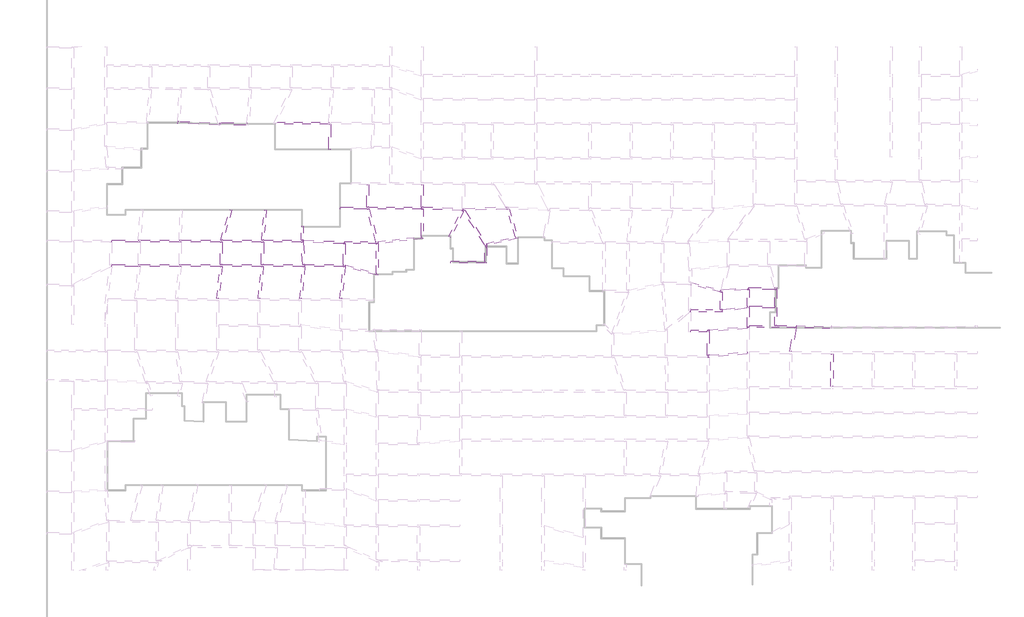
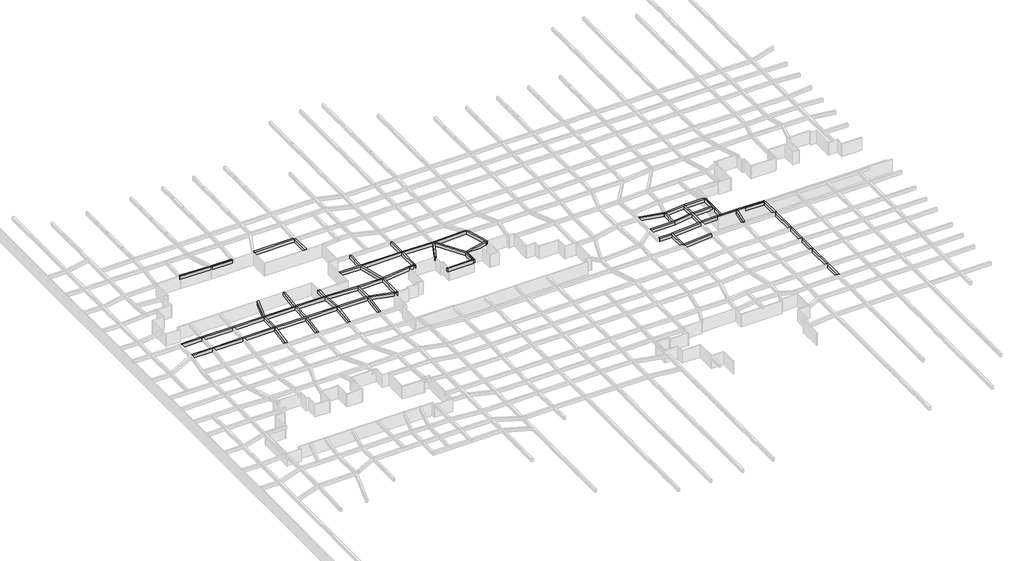
# One storey, part 30 of 45: 53 beams.
"""IFC4 building model written with IfcOpenShell, lengths in millimetres."""

import ifcopenshell
import ifcopenshell.guid

model = None  # the IFC model being written
_history = None  # IfcOwnerHistory: only IFC2X3 demands one
_inside = {}  # id of a spatial element -> (the spatial element, [elements in it])
_under = {}  # id of a project, library or spatial element -> (it, [spatial elements below it])
_declared = {}  # id of a project -> (the project, [libraries it declares])
_typed = {}  # id of a type object -> (the type object, [elements of that type])
_made_of = {}  # id of a material, layer set ... -> (it, [elements and type objects made of it])


def new_model(schema):
    """Start an empty IFC model of exactly this schema.

    Asked for "IFC4X3", IfcOpenShell would pick the latest addendum, in which some entities
    have other attributes; the version numbers below select the first issue.
    IFC2X3 requires an IfcOwnerHistory on every rooted entity: one is made here for all.
    """
    global model, _history
    if schema == "IFC4X3":
        model = ifcopenshell.file(schema_version=(4, 3, 0, 0))
    else:
        model = ifcopenshell.file(schema=schema)
    _inside.clear()
    _under.clear()
    _declared.clear()
    _typed.clear()
    _made_of.clear()
    _history = None
    if model.schema == "IFC2X3":
        org = make("IfcOrganization", Name="unknown")
        user = make(
            "IfcPersonAndOrganization",
            ThePerson=make("IfcPerson", FamilyName="unknown"),
            TheOrganization=org,
        )
        app = make(
            "IfcApplication",
            ApplicationDeveloper=org,
            Version="unknown",
            ApplicationFullName="unknown",
            ApplicationIdentifier="unknown",
        )
        _history = make(
            "IfcOwnerHistory",
            OwningUser=user,
            OwningApplication=app,
            ChangeAction="ADDED",
            CreationDate=0,
        )
    return model


def make(cls, **values):
    """One entity of the class cls with the attributes given. An attribute that is None is left unset."""
    return model.create_entity(
        cls, **{name: value for name, value in values.items() if value is not None}
    )


def rooted(cls, **values):
    """An entity with a GlobalId (a new one), such as an element, a storey or a relation."""
    return make(cls, GlobalId=ifcopenshell.guid.new(), OwnerHistory=_history, **values)


def si_unit(unit_type, name, prefix=None):
    """IfcSIUnit, for example si_unit("LENGTHUNIT", "METRE", prefix="MILLI")."""
    return make("IfcSIUnit", UnitType=unit_type, Prefix=prefix, Name=name)


def assignment(units):
    """IfcUnitAssignment: the units of a project."""
    return None if units is None else make("IfcUnitAssignment", Units=units)


def point(xyz):
    """IfcCartesianPoint."""
    return None if xyz is None else make("IfcCartesianPoint", Coordinates=xyz)


def direction(xyz):
    """IfcDirection."""
    return None if xyz is None else make("IfcDirection", DirectionRatios=xyz)


def frame(location, z_axis=None, x_axis=None):
    """IfcAxis2Placement3D, a coordinate frame: its origin and axes. An axis left out is left unset."""
    return make(
        "IfcAxis2Placement3D",
        Location=point(location),
        Axis=direction(z_axis),
        RefDirection=direction(x_axis),
    )


def origin():
    """The frame at (0, 0, 0) with its axes left unset."""
    return frame((0.0, 0.0, 0.0))


def place(relative_to, where):
    """IfcLocalPlacement: puts the frame where relative to a parent placement (None: the world)."""
    return make(
        "IfcLocalPlacement", PlacementRelTo=relative_to, RelativePlacement=where
    )


def context(
    kind, dimensions, precision=None, world=None, true_north=None, identifier=None
):
    """IfcGeometricRepresentationContext, for example the 3D "Model" context."""
    return make(
        "IfcGeometricRepresentationContext",
        ContextIdentifier=identifier,
        ContextType=kind,
        CoordinateSpaceDimension=dimensions,
        Precision=precision,
        WorldCoordinateSystem=world,
        TrueNorth=true_north,
    )


def project(units=None, contexts=None):
    """IfcProject with its units and contexts."""
    return rooted(
        "IfcProject",
        Name="project",
        RepresentationContexts=contexts,
        UnitsInContext=assignment(units),
    )


def spatial(cls, under=None, at=None, **own):
    """A site, building, storey or space (cls), placed at a placement, below another one or the project."""
    s = rooted(cls, ObjectPlacement=at, **own)
    if under is not None:
        _under.setdefault(under.id(), (under, []))[1].append(s)
    return s


def polyline(points):
    """IfcPolyline through the points."""
    return make("IfcPolyline", Points=[point(p) for p in points])


def outline(outer, holes=None, kind="AREA"):
    """IfcArbitraryClosedProfileDef: a profile drawn as a closed curve; with holes, ...WithVoids."""
    if holes is None:
        return make("IfcArbitraryClosedProfileDef", ProfileType=kind, OuterCurve=outer)
    return make(
        "IfcArbitraryProfileDefWithVoids",
        ProfileType=kind,
        OuterCurve=outer,
        InnerCurves=holes,
    )


def extrude(swept, where, along, depth):
    """IfcExtrudedAreaSolid: the profile swept, set in the frame where, extruded along a direction by depth."""
    return make(
        "IfcExtrudedAreaSolid",
        SweptArea=swept,
        Position=where,
        ExtrudedDirection=direction(along),
        Depth=depth,
    )


def faces_of(points, faces, orient=None, outer=None):
    """IfcFace entities. A face is a list of loops; a loop is a list of indices into points, from 0.

    orient and outer hold one flag for each loop. By default every Orientation is true, the
    first loop of a face is its IfcFaceOuterBound and the others are IfcFaceBound.
    """
    made = []
    for i, loops in enumerate(faces):
        bounds = []
        for j, loop in enumerate(loops):
            is_outer = j == 0 if outer is None else outer[i][j]
            bounds.append(
                make(
                    "IfcFaceOuterBound" if is_outer else "IfcFaceBound",
                    Bound=make("IfcPolyLoop", Polygon=[points[k] for k in loop]),
                    Orientation=True if orient is None else orient[i][j],
                )
            )
        made.append(make("IfcFace", Bounds=bounds))
    return made


def faceted_brep(points, faces, orient=None, outer=None, voids=None):
    """IfcFacetedBrep: a solid bounded by flat faces; with voids (closed shells), ...WithVoids."""
    shared = [point(p) for p in points]
    hull = make("IfcClosedShell", CfsFaces=faces_of(shared, faces, orient, outer))
    if voids is None:
        return make("IfcFacetedBrep", Outer=hull)
    return make(
        "IfcFacetedBrepWithVoids",
        Outer=hull,
        Voids=[
            make(cls, CfsFaces=faces_of(shared, fs, o, b)) for cls, fs, o, b in voids
        ],
    )


def shape(context_of_items, identifier, shape_type, items):
    """IfcShapeRepresentation: the items that make up one representation, for example the "Body"."""
    return make(
        "IfcShapeRepresentation",
        ContextOfItems=context_of_items,
        RepresentationIdentifier=identifier,
        RepresentationType=shape_type,
        Items=items,
    )


def made_of(thing, what):
    """Note that an element or type object is made of a material, layer set ...; save() writes the relation."""
    if what is not None:
        _made_of.setdefault(what.id(), (what, []))[1].append(thing)
    return thing


def element(
    cls,
    number,
    at=None,
    inside=None,
    cuts=None,
    type_object=None,
    material=None,
    context=None,
    identifier="Body",
    shape_type=None,
    held_by="IfcProductDefinitionShape",
    body=None,
    shapes=None,
    **own,
):
    """One element of the class cls, such as IfcWall. Its Tag is "e" and its number.

    at: its placement. inside: the storey or other place that contains it. cuts: it is an
    opening in that element (IfcRelVoidsElement). A single representation is given by context,
    identifier, shape_type and body (its items); several are given by shapes. held_by: the class
    of the entity that holds the representations. save() writes the other relations.
    """
    e = rooted(cls, Tag="e%d" % number, ObjectPlacement=at, **own)
    if body is not None:
        shapes = [shape(context, identifier, shape_type, body)]
    if shapes is not None:
        e.Representation = make(held_by, Representations=shapes)
    if inside is not None:
        _inside.setdefault(inside.id(), (inside, []))[1].append(e)
    if cuts is not None:
        rooted(
            "IfcRelVoidsElement", RelatingBuildingElement=cuts, RelatedOpeningElement=e
        )
    if type_object is not None:
        _typed.setdefault(type_object.id(), (type_object, []))[1].append(e)
    return made_of(e, material)


def aggregate(whole, parts):
    """IfcRelAggregates: a whole, such as a stair, and the parts it consists of."""
    return rooted("IfcRelAggregates", RelatingObject=whole, RelatedObjects=parts)


def save(model, path):
    """Write the relations noted so far, then the file.

    IfcRelAggregates (storeys below a building ...), IfcRelContainedInSpatialStructure (elements
    in a storey), IfcRelDefinesByType, IfcRelAssociatesMaterial and IfcRelDeclares: one each for
    every whole, place, type object, material and project.
    """
    for whole, parts in _under.values():
        aggregate(whole, parts)
    for where, things in _inside.values():
        rooted(
            "IfcRelContainedInSpatialStructure",
            RelatedElements=things,
            RelatingStructure=where,
        )
    for kind, things in _typed.values():
        rooted("IfcRelDefinesByType", RelatedObjects=things, RelatingType=kind)
    for what, things in _made_of.values():
        rooted("IfcRelAssociatesMaterial", RelatedObjects=things, RelatingMaterial=what)
    for by, libraries in _declared.values():
        rooted("IfcRelDeclares", RelatingContext=by, RelatedDefinitions=libraries)
    model.write(path)


model = new_model("IFC4")

# Units and contexts
model_context = context("Model", 3, world=origin())
ifc_project = project(units=[si_unit("LENGTHUNIT", "METRE", prefix="MILLI")], contexts=[model_context])

# Site, building, storey
site = spatial("IfcSite", under=ifc_project)
building = spatial("IfcBuilding", under=site)
storey = spatial("IfcBuildingStorey", under=building, Name="户型图", Elevation=0.0)

# Beams
placement = place(None, origin())
element("IfcBeam", 1, ObjectType="混凝土 - 矩形梁 : KL_beam", at=placement, inside=storey, context=model_context, shape_type="Brep", body=[
    faceted_brep([(-106255.594098, 67607.285668, 3300.0), (-106259.7681682, 67607.285668, 3300.0), (-106661.2961032, 67607.285668, 3300.0), (-114062.8131158, 67607.285668, 3300.0), (-114464.9837666, 67607.285668, 3300.0), (-121862.8299892, 67607.285668, 3300.0), (-122265.00064, 67607.285668, 3300.0), (-129662.8131158, 67607.285668, 3300.0), (-130064.9837666, 67607.285668, 3300.0), (-137362.8299892, 67607.285668, 3300.0), (-137765.00064, 67607.285668, 3300.0), (-142766.12907, 67607.285668, 3300.0), (-142895.0186512, 67607.285668, 3300.0), (-142895.0186512, 67607.285668, 2500.0), (-142766.12907, 67607.285668, 2500.0), (-137765.00064, 67607.285668, 2500.0), (-137362.8299892, 67607.285668, 2500.0), (-130064.9837666, 67607.285668, 2500.0), (-129662.8131158, 67607.285668, 2500.0), (-122265.00064, 67607.285668, 2500.0), (-121862.8299892, 67607.285668, 2500.0), (-114464.9837666, 67607.285668, 2500.0), (-114062.8131158, 67607.285668, 2500.0), (-106661.2961032, 67607.285668, 2500.0), (-106259.7681682, 67607.285668, 2500.0), (-106255.594098, 67607.285668, 2500.0), (-142743.034403, 67684.7255104, 3300.0), (-142743.034403, 67684.7255104, 2500.0), (-142743.034403, 68007.285668, 3300.0), (-142743.034403, 68007.285668, 2500.0), (-106255.594098, 68007.285668, 3300.0), (-106656.4356776, 68007.285668, 3300.0), (-114043.034403, 68007.285668, 3300.0), (-114443.034403, 68007.285668, 3300.0), (-121843.034403, 68007.285668, 3300.0), (-122243.034403, 68007.285668, 3300.0), (-129643.034403, 68007.285668, 3300.0), (-130043.034403, 68007.285668, 3300.0), (-137343.034403, 68007.285668, 3300.0), (-137743.034403, 68007.285668, 3300.0), (-137743.034403, 68007.285668, 2500.0), (-137343.034403, 68007.285668, 2500.0), (-130043.034403, 68007.285668, 2500.0), (-129643.034403, 68007.285668, 2500.0), (-122243.034403, 68007.285668, 2500.0), (-121843.034403, 68007.285668, 2500.0), (-114443.034403, 68007.285668, 2500.0), (-114043.034403, 68007.285668, 2500.0), (-106656.4356776, 68007.285668, 2500.0), (-106255.594098, 68007.285668, 2500.0)], [[[0, 1, 2, 3, 4, 5, 6, 7, 8, 9, 10, 11, 12, 13, 14, 15, 16, 17, 18, 19, 20, 21, 22, 23, 24, 25]], [[26, 27, 13, 12]], [[27, 26, 28, 29]], [[30, 31, 32, 33, 34, 35, 36, 37, 38, 39, 28, 26, 12, 11, 10, 9, 8, 7, 6, 5, 4, 3, 2, 1, 0]], [[25, 24, 23, 22, 21, 20, 19, 18, 17, 16, 15, 14, 13, 27, 29, 40, 41, 42, 43, 44, 45, 46, 47, 48, 49]], [[28, 39, 38, 37, 36, 35, 34, 33, 32, 31, 30, 49, 48, 47, 46, 45, 44, 43, 42, 41, 40, 29]], [[30, 0, 25, 49]]]),
])
element("IfcBeam", 2, ObjectType="混凝土 - 矩形梁 : KL_beam", at=placement, inside=storey, context=model_context, shape_type="Brep", body=[
    faceted_brep([(-142743.034403, 72629.6091605, 3300.0), (-142743.034403, 72229.932653, 3300.0), (-142743.034403, 72229.6091605, 3300.0), (-137743.034403, 72229.6091605, 3300.0), (-137343.034403, 72229.6091605, 3300.0), (-130043.034403, 72229.6091605, 3300.0), (-129643.034403, 72229.6091605, 3300.0), (-122243.034403, 72229.6091605, 3300.0), (-121843.034403, 72229.6091605, 3300.0), (-114443.034403, 72229.6091605, 3300.0), (-114043.034403, 72229.6091605, 3300.0), (-106930.474708, 72229.6091605, 3300.0), (-106529.6331284, 72229.6091605, 3300.0), (-106543.0328284, 72436.0683208, 3300.0), (-106555.594098, 72629.6091605, 3300.0), (-106943.0328284, 72629.6091605, 3300.0), (-114024.7727028, 72629.6091605, 3300.0), (-114426.3006378, 72629.6091605, 3300.0), (-121772.7499154, 72629.6091605, 3300.0), (-122191.026618, 72629.6091605, 3300.0), (-129635.9283402, 72629.6091605, 3300.0), (-130036.172158, 72629.6091605, 3300.0), (-137328.560661, 72629.6091605, 3300.0), (-137729.5374202, 72629.6091605, 3300.0), (-106529.6331284, 72229.6091605, 2500.0), (-142743.034403, 72229.6091605, 2500.0), (-137743.034403, 72229.6091605, 2500.0), (-137343.034403, 72229.6091605, 2500.0), (-130043.034403, 72229.6091605, 2500.0), (-129643.034403, 72229.6091605, 2500.0), (-122243.034403, 72229.6091605, 2500.0), (-121843.034403, 72229.6091605, 2500.0), (-114443.034403, 72229.6091605, 2500.0), (-114043.034403, 72229.6091605, 2500.0), (-106930.474708, 72229.6091605, 2500.0), (-142743.034403, 72229.932653, 2500.0), (-142743.034403, 72629.6091605, 2500.0), (-137729.5374202, 72629.6091605, 2500.0), (-137328.560661, 72629.6091605, 2500.0), (-130036.172158, 72629.6091605, 2500.0), (-129635.9283402, 72629.6091605, 2500.0), (-122191.026618, 72629.6091605, 2500.0), (-121772.7499154, 72629.6091605, 2500.0), (-114426.3006378, 72629.6091605, 2500.0), (-114024.7727028, 72629.6091605, 2500.0), (-106943.0328284, 72629.6091605, 2500.0), (-106555.594098, 72629.6091605, 2500.0), (-106543.0328284, 72436.0683208, 2500.0)], [[[0, 1, 2, 3, 4, 5, 6, 7, 8, 9, 10, 11, 12, 13, 14, 15, 16, 17, 18, 19, 20, 21, 22, 23]], [[24, 12, 11, 10, 9, 8, 7, 6, 5, 4, 3, 2, 25, 26, 27, 28, 29, 30, 31, 32, 33, 34]], [[25, 35, 36, 37, 38, 39, 40, 41, 42, 43, 44, 45, 46, 47, 24, 34, 33, 32, 31, 30, 29, 28, 27, 26]], [[36, 0, 23, 22, 21, 20, 19, 18, 17, 16, 15, 14, 46, 45, 44, 43, 42, 41, 40, 39, 38, 37]], [[0, 36, 35, 25, 2, 1]], [[14, 13, 12, 24, 47, 46]]]),
])
element("IfcBeam", 3, ObjectType="混凝土 - 矩形梁 : KL_beam", at=placement, inside=storey, context=model_context, shape_type="SweptSolid", body=[
    extrude(outline(polyline([(-121843.034403, 68007.285668), (-122243.034403, 68007.285668), (-122243.034403, 72229.6091605), (-121843.034403, 72229.6091605), (-121843.034403, 68007.285668)])), frame((0.0, 0.0, 2500.0), z_axis=(0.0, 0.0, 1.0), x_axis=(1.0, 0.0, 0.0)), (0.0, 0.0, 1.0), 800.0),
])
element("IfcBeam", 4, ObjectType="混凝土 - 矩形梁 : KL_beam", at=placement, inside=storey, context=model_context, shape_type="SweptSolid", body=[
    extrude(outline(polyline([(-114043.034403, 68007.285668), (-114443.034403, 68007.285668), (-114443.034403, 72229.6091605), (-114043.034403, 72229.6091605), (-114043.034403, 68007.285668)])), frame((0.0, 0.0, 2500.0), z_axis=(0.0, 0.0, 1.0), x_axis=(1.0, 0.0, 0.0)), (0.0, 0.0, 1.0), 800.0),
])
element("IfcBeam", 5, ObjectType="混凝土 - 矩形梁 : KL_beam", at=placement, inside=storey, context=model_context, shape_type="Brep", body=[
    faceted_brep([(-106656.4356776, 68007.285668, 3300.0), (-106255.594098, 68007.285668, 3300.0), (-106529.1388631, 72221.9936481, 3300.0), (-106529.6331284, 72229.6091605, 3300.0), (-106930.474708, 72229.6091605, 3300.0), (-106229.6331284, 67607.285668, 3300.0), (-106229.6331284, 67607.285668, 2500.0), (-106255.594098, 68007.285668, 2500.0), (-106529.1388631, 72221.9936481, 2500.0), (-106529.6331284, 72229.6091605, 2500.0), (-106656.4356776, 68007.285668, 2500.0), (-106930.474708, 72229.6091605, 2500.0), (-106255.594098, 67607.285668, 3300.0), (-106255.594098, 67607.285668, 2500.0)], [[[0, 1, 2, 3, 4]], [[5, 6, 7, 8, 9, 3, 2, 1]], [[7, 10, 11, 9, 8]], [[10, 0, 4, 11]], [[6, 5, 12, 13]], [[7, 1, 0, 10]], [[1, 7, 13, 12]], [[12, 5, 1]], [[6, 13, 7]], [[4, 3, 9, 11]]]),
])
element("IfcBeam", 6, ObjectType="混凝土 - 矩形梁 : KL_beam", at=placement, inside=storey, context=model_context, shape_type="SweptSolid", body=[
    extrude(outline(polyline([(-120421.5907849, 78417.1729884), (-120039.0688825, 78300.2243065), (-121772.7499154, 72629.6091605), (-122191.026618, 72629.6091605), (-120421.5907849, 78417.1729884)])), frame((0.0, 0.0, 2500.0), z_axis=(0.0, 0.0, 1.0), x_axis=(1.0, 0.0, 0.0)), (0.0, 0.0, 1.0), 800.0),
])
element("IfcBeam", 7, ObjectType="混凝土 - 矩形梁 : KL_beam", at=placement, inside=storey, context=model_context, shape_type="SweptSolid", body=[
    extrude(outline(polyline([(-113928.0544604, 78324.5890278), (-113529.5765812, 78289.7267307), (-114024.7727028, 72629.6091605), (-114426.3006378, 72629.6091605), (-113928.0544604, 78324.5890278)])), frame((0.0, 0.0, 2500.0), z_axis=(0.0, 0.0, 1.0), x_axis=(1.0, 0.0, 0.0)), (0.0, 0.0, 1.0), 800.0),
])
element("IfcBeam", 8, ObjectType="混凝土 - 矩形梁 : KL_beam", at=placement, inside=storey, context=model_context, shape_type="Brep", body=[
    faceted_brep([(-106943.0328284, 75329.5848988, 3300.0), (-106543.0328284, 75329.5848988, 3300.0), (-106543.0328284, 75329.5848988, 2500.0), (-106943.0328284, 75329.5848988, 2500.0), (-106943.0328284, 72629.6091605, 3300.0), (-106555.594098, 72629.6091605, 3300.0), (-106543.0328284, 72436.0683208, 3300.0), (-106543.0328284, 72622.7226537, 3300.0), (-106543.0328284, 72436.0683208, 2500.0), (-106543.0328284, 72622.7226537, 2500.0), (-106555.594098, 72629.6091605, 2500.0), (-106943.0328284, 72629.6091605, 2500.0)], [[[0, 1, 2, 3]], [[1, 0, 4, 5, 6, 7]], [[2, 1, 7, 6, 8, 9]], [[3, 2, 9, 8, 10, 11]], [[0, 3, 11, 4]], [[5, 10, 8, 6]], [[10, 5, 4, 11]]]),
])
element("IfcBeam", 9, ObjectType="混凝土 - 矩形梁 : KL_beam", at=placement, inside=storey, context=model_context, shape_type="SweptSolid", body=[
    extrude(outline(polyline([(-111770.1722019, 94559.1732079), (-111583.6491387, 94959.1732079), (-101725.1277611, 94959.1732079), (-101753.0984859, 94559.1732079), (-111770.1722019, 94559.1732079)])), frame((0.0, 0.0, 2500.0), z_axis=(0.0, 0.0, 1.0), x_axis=(1.0, 0.0, 0.0)), (0.0, 0.0, 1.0), 800.0),
])
element("IfcBeam", 10, ObjectType="混凝土 - 矩形梁 : KL_beam", at=placement, inside=storey, context=model_context, shape_type="Brep", body=[
    faceted_brep([(-101338.6349683, 89759.1001002, 3300.0), (-101738.6349683, 89759.1001002, 3300.0), (-101738.6349683, 89759.1001002, 2500.0), (-101338.6349683, 89759.1001002, 2500.0), (-101338.6349683, 94559.0757309, 3300.0), (-101352.1285421, 94559.0790192, 3300.0), (-101738.6349683, 94559.1732079, 3300.0), (-101738.6349683, 94559.1732079, 2500.0), (-101352.1285421, 94559.0790192, 2500.0), (-101338.6349683, 94559.0757309, 2500.0)], [[[0, 1, 2, 3]], [[1, 0, 4, 5, 6]], [[2, 1, 6, 7]], [[3, 2, 7, 8, 9]], [[0, 3, 9, 4]], [[4, 9, 8, 7, 6, 5]]]),
])
element("IfcBeam", 11, ObjectType="混凝土 - 矩形梁 : KL_beam", at=placement, inside=storey, context=model_context, shape_type="SweptSolid", body=[
    extrude(outline(polyline([(-122119.8995169, 94446.2535162), (-122242.1917895, 94846.2535162), (-117187.4621963, 94846.2535162), (-117215.4329211, 94446.2535162), (-122119.8995169, 94446.2535162)])), frame((0.0, 0.0, 2500.0), z_axis=(0.0, 0.0, 1.0), x_axis=(1.0, 0.0, 0.0)), (0.0, 0.0, 1.0), 800.0),
])
element("IfcBeam", 12, ObjectType="混凝土 - 矩形梁 : KL_beam", at=placement, inside=storey, context=model_context, shape_type="Brep", body=[
    faceted_brep([(-122397.9223476, 94446.3883014, 3300.0), (-122397.9223476, 94446.3883014, 2500.0), (-122383.9625489, 94846.1446322, 2500.0), (-122383.9625489, 94846.1446322, 3300.0), (-129850.782274, 95106.8917227, 3300.0), (-130250.5386048, 95120.8515214, 3300.0), (-130264.4984035, 94721.0951906, 3300.0), (-129850.782274, 95106.8917227, 2500.0), (-130250.5386048, 95120.8515214, 2500.0), (-130264.4984035, 94721.0951906, 2500.0)], [[[0, 1, 2, 3]], [[0, 3, 4, 5, 6]], [[3, 2, 7, 8, 5, 4]], [[2, 1, 9, 8, 7]], [[1, 0, 6, 9]], [[6, 5, 8, 9]]]),
])
element("IfcBeam", 13, ObjectType="混凝土 - 矩形梁 : KL_beam", at=placement, inside=storey, context=model_context, shape_type="Brep", body=[
    faceted_brep([(-76269.0646381, 78646.8472266, 3300.0), (-76269.0646381, 78246.6034089, 3300.0), (-75912.1939504, 78259.0656079, 3300.0), (-68020.5737025, 78534.6470595, 3300.0), (-67874.1816912, 78539.7591812, 3300.0), (-67874.1816912, 78940.0029989, 3300.0), (-68231.227169, 78927.5346961, 3300.0), (-76029.0040152, 78655.2303283, 3300.0), (-76269.0646381, 78646.8472266, 2500.0), (-67874.1816912, 78940.0029989, 2500.0), (-68231.227169, 78927.5346961, 2500.0), (-76029.0040152, 78655.2303283, 2500.0), (-76269.0646381, 78246.6034089, 2500.0), (-67874.1816912, 78539.7591812, 2500.0), (-68020.5737025, 78534.6470595, 2500.0), (-75912.1939504, 78259.0656079, 2500.0)], [[[0, 1, 2, 3, 4, 5, 6, 7]], [[8, 0, 7, 6, 5, 9, 10, 11]], [[12, 8, 11, 10, 9, 13, 14, 15]], [[1, 12, 15, 14, 13, 4, 3, 2]], [[4, 13, 9, 5]], [[1, 0, 8, 12]]]),
])
element("IfcBeam", 14, ObjectType="混凝土 - 矩形梁 : KL_beam", at=placement, inside=storey, context=model_context, shape_type="Brep", body=[
    faceted_brep([(-76269.0646381, 78246.6034089, 3300.0), (-76269.0646381, 78646.8472266, 3300.0), (-76429.0040152, 78652.4324327, 3300.0), (-83861.6804358, 78911.9872127, 3300.0), (-84261.6804358, 78925.9555205, 3300.0), (-84261.6804358, 78918.8494577, 3300.0), (-84261.6804358, 78525.7117028, 3300.0), (-84065.1714488, 78518.8494577, 3300.0), (-83862.0339972, 78511.7557416, 3300.0), (-76584.1894618, 78257.6078102, 3300.0), (-76381.2779443, 78250.5219839, 3300.0), (-76269.0646381, 78646.8472266, 2500.0), (-76429.0040152, 78652.4324327, 2500.0), (-83861.6804358, 78911.9872127, 2500.0), (-84261.6804358, 78925.9555205, 2500.0), (-76269.0646381, 78246.6034089, 2500.0), (-76381.2779443, 78250.5219839, 2500.0), (-76584.1894618, 78257.6078102, 2500.0), (-83862.0339972, 78511.7557416, 2500.0), (-84065.1714488, 78518.8494577, 2500.0), (-84261.6804358, 78525.7117028, 2500.0), (-84261.6804358, 78918.8494577, 2500.0)], [[[0, 1, 2, 3, 4, 5, 6, 7, 8, 9, 10]], [[1, 11, 12, 13, 14, 4, 3, 2]], [[11, 15, 16, 17, 18, 19, 20, 21, 14, 13, 12]], [[15, 0, 10, 9, 8, 7, 6, 20, 19, 18, 17, 16]], [[0, 15, 11, 1]], [[6, 5, 4, 14, 21, 20]]]),
])
element("IfcBeam", 15, ObjectType="混凝土 - 矩形梁 : KL_beam", at=placement, inside=storey, context=model_context, shape_type="SweptSolid", body=[
    extrude(outline(polyline([(-83861.6804358, 78911.9872127), (-84261.6804358, 78925.9555205), (-84261.6804358, 83154.2865852), (-83861.6804358, 83154.2865852), (-83861.6804358, 78911.9872127)])), frame((0.0, 0.0, 2500.0), z_axis=(0.0, 0.0, 1.0), x_axis=(1.0, 0.0, 0.0)), (0.0, 0.0, 1.0), 800.0),
])
element("IfcBeam", 16, ObjectType="混凝土 - 矩形梁 : KL_beam", at=placement, inside=storey, context=model_context, shape_type="Brep", body=[
    faceted_brep([(-99591.0339972, 78518.8494577, 3300.0), (-99591.0339972, 78918.8494577, 3300.0), (-99591.0339972, 78918.8494577, 2500.0), (-99591.0339972, 78518.8494577, 2500.0), (-94484.7943922, 78518.8494577, 3300.0), (-94070.68392, 78518.8494577, 3300.0), (-84262.0339972, 78518.8494577, 3300.0), (-84065.1714488, 78518.8494577, 3300.0), (-84261.6804358, 78525.7117028, 3300.0), (-84261.6804358, 78918.8494577, 3300.0), (-94131.3875586, 78918.8494577, 3300.0), (-94531.3875586, 78918.8494577, 3300.0), (-84261.6804358, 78918.8494577, 2500.0), (-94131.3875586, 78918.8494577, 2500.0), (-94531.3875586, 78918.8494577, 2500.0), (-84261.6804358, 78525.7117028, 2500.0), (-84065.1714488, 78518.8494577, 2500.0), (-84262.0339972, 78518.8494577, 2500.0), (-94070.68392, 78518.8494577, 2500.0), (-94484.7943922, 78518.8494577, 2500.0)], [[[0, 1, 2, 3]], [[1, 0, 4, 5, 6, 7, 8, 9, 10, 11]], [[2, 1, 11, 10, 9, 12, 13, 14]], [[3, 2, 14, 13, 12, 15, 16, 17, 18, 19]], [[0, 3, 19, 18, 17, 16, 7, 6, 5, 4]], [[15, 8, 7, 16]], [[8, 15, 12, 9]]]),
])
element("IfcBeam", 17, ObjectType="混凝土 - 矩形梁 : KL_beam", at=placement, inside=storey, context=model_context, shape_type="SweptSolid", body=[
    extrude(outline(polyline([(-94531.3875586, 83154.2865852), (-94131.3875586, 83154.2865852), (-94131.3875586, 78918.8494577), (-94531.3875586, 78918.8494577), (-94531.3875586, 83154.2865852)])), frame((0.0, 0.0, 2500.0), z_axis=(0.0, 0.0, 1.0), x_axis=(1.0, 0.0, 0.0)), (0.0, 0.0, 1.0), 800.0),
])
element("IfcBeam", 18, ObjectType="混凝土 - 矩形梁 : KL_beam", at=placement, inside=storey, context=model_context, shape_type="Brep", body=[
    faceted_brep([(-29976.7146993, 50850.070339, 3300.0), (-29959.2503222, 50450.070339, 3300.0), (-29767.9825107, 50466.8041042, 3300.0), (-22564.0859234, 51097.0633889, 3300.0), (-22564.0859234, 51498.5913239, 3300.0), (-29767.9825107, 50868.3320393, 3300.0), (-29959.2503222, 50450.070339, 2500.0), (-29767.9825107, 50466.8041042, 2500.0), (-22564.0859234, 51097.0633889, 2500.0), (-29976.7146993, 50850.070339, 2500.0), (-29767.9825107, 50868.3320393, 2500.0), (-22564.0859234, 51498.5913239, 2500.0)], [[[0, 1, 2, 3, 4, 5]], [[1, 6, 7, 8, 3, 2]], [[6, 9, 10, 11, 8, 7]], [[9, 0, 5, 4, 11, 10]], [[0, 9, 6, 1]], [[4, 3, 8, 11]]]),
])
element("IfcBeam", 19, ObjectType="混凝土 - 矩形梁 : KL_beam", at=placement, inside=storey, context=model_context, shape_type="Brep", body=[
    faceted_brep([(-30167.9825107, 50850.070339, 3300.0), (-29976.7146993, 50850.070339, 3300.0), (-29767.9825107, 50868.3320393, 3300.0), (-29767.9825107, 55266.8041042, 3300.0), (-29767.9825107, 55650.070339, 3300.0), (-29976.7146993, 55650.070339, 3300.0), (-30167.9825107, 55650.070339, 3300.0), (-30167.9825107, 55250.070339, 3300.0), (-29767.9825107, 55650.070339, 2500.0), (-29767.9825107, 50868.3320393, 2500.0), (-29767.9825107, 55266.8041042, 2500.0), (-29976.7146993, 50850.070339, 2500.0), (-30167.9825107, 50850.070339, 2500.0), (-30167.9825107, 55250.070339, 2500.0), (-30167.9825107, 55650.070339, 2500.0), (-29976.7146993, 55650.070339, 2500.0)], [[[0, 1, 2, 3, 4, 5, 6, 7]], [[8, 4, 3, 2, 9, 10]], [[11, 12, 13, 14, 15, 8, 10, 9]], [[12, 0, 7, 6, 14, 13]], [[1, 0, 12, 11]], [[2, 1, 11, 9]], [[6, 5, 4, 8, 15, 14]]]),
])
element("IfcBeam", 20, ObjectType="混凝土 - 矩形梁 : KL_beam", at=placement, inside=storey, context=model_context, shape_type="Brep", body=[
    faceted_brep([(-65916.2620344, 73019.8751777, 3300.0), (-67600.9427374, 78530.2174666, 3300.0), (-67874.1816912, 78539.7591812, 3300.0), (-67981.3269257, 78536.0175871, 3300.0), (-68020.5737025, 78534.6470595, 3300.0), (-66416.0181954, 73286.3824777, 3300.0), (-66298.7839367, 72902.9264958, 3300.0), (-68020.5737025, 78534.6470595, 2500.0), (-66416.0181954, 73286.3824777, 2500.0), (-66298.7839367, 72902.9264958, 2500.0), (-67600.9427374, 78530.2174666, 2500.0), (-65916.2620344, 73019.8751777, 2500.0), (-67981.3269257, 78536.0175871, 2500.0), (-67874.1816912, 78539.7591812, 2500.0)], [[[0, 1, 2, 3, 4, 5, 6]], [[6, 5, 4, 7, 8, 9]], [[10, 11, 9, 8, 7, 12, 13]], [[1, 0, 11, 10]], [[2, 1, 10, 13]], [[7, 4, 3, 2, 13, 12]], [[0, 6, 9, 11]]]),
])
element("IfcBeam", 21, ObjectType="混凝土 - 矩形梁 : KL_beam", at=placement, inside=storey, context=model_context, shape_type="Brep", body=[
    faceted_brep([(-76269.0646381, 78246.6034089, 3300.0), (-76381.2779443, 78250.5219839, 3300.0), (-76245.9854172, 78038.560049, 3300.0), (-72218.8192159, 71729.2245821, 3300.0), (-71818.8192159, 71102.5471468, 3300.0), (-71818.8192159, 71628.5259359, 3300.0), (-71818.8192159, 71846.0016564, 3300.0), (-71926.2124219, 72014.2539038, 3300.0), (-75912.1939504, 78259.0656079, 3300.0), (-76029.0040152, 78254.9865105, 3300.0), (-76381.2779443, 78250.5219839, 2500.0), (-76245.9854172, 78038.560049, 2500.0), (-72218.8192159, 71729.2245821, 2500.0), (-71818.8192159, 71102.5471468, 2500.0), (-76269.0646381, 78246.6034089, 2500.0), (-76029.0040152, 78254.9865105, 2500.0), (-75912.1939504, 78259.0656079, 2500.0), (-71926.2124219, 72014.2539038, 2500.0), (-71818.8192159, 71846.0016564, 2500.0), (-71818.8192159, 71628.5259359, 2500.0)], [[[0, 1, 2, 3, 4, 5, 6, 7, 8, 9]], [[1, 10, 11, 12, 13, 4, 3, 2]], [[10, 14, 15, 16, 17, 18, 19, 13, 12, 11]], [[16, 8, 7, 6, 18, 17]], [[1, 0, 14, 10]], [[8, 16, 15, 14, 0, 9]], [[6, 5, 4, 13, 19, 18]]]),
])
element("IfcBeam", 22, ObjectType="混凝土 - 矩形梁 : KL_beam", at=placement, inside=storey, context=model_context, shape_type="Brep", body=[
    faceted_brep([(-72218.8192159, 68287.6131193, 3300.0), (-71818.8192159, 68287.6131193, 3300.0), (-71818.8192159, 71102.5471468, 3300.0), (-72218.8192159, 71729.2245821, 3300.0), (-72218.8192159, 68687.6131193, 3300.0), (-72218.8192159, 68287.6131193, 2500.0), (-72218.8192159, 71729.2245821, 2500.0), (-72218.8192159, 68687.6131193, 2500.0), (-71818.8192159, 68287.6131193, 2500.0), (-71818.8192159, 71102.5471468, 2500.0)], [[[0, 1, 2, 3, 4]], [[5, 0, 4, 3, 6, 7]], [[8, 5, 7, 6, 9]], [[1, 8, 9, 2]], [[3, 2, 9, 6]], [[1, 0, 5, 8]]]),
])
element("IfcBeam", 23, ObjectType="混凝土 - 矩形梁 : KL_beam", at=placement, inside=storey, context=model_context, shape_type="SweptSolid", body=[
    extrude(outline(polyline([(-78618.8192159, 68287.6131193), (-78618.8192159, 68687.6131193), (-72218.8192159, 68687.6131193), (-72218.8192159, 68287.6131193), (-78618.8192159, 68287.6131193)])), frame((0.0, 0.0, 2500.0), z_axis=(0.0, 0.0, 1.0), x_axis=(1.0, 0.0, 0.0)), (0.0, 0.0, 1.0), 800.0),
])
element("IfcBeam", 24, ObjectType="混凝土 - 矩形梁 : KL_beam", at=placement, inside=storey, context=model_context, shape_type="Brep", body=[
    faceted_brep([(-84262.0339972, 72894.8122003, 3300.0), (-83862.0339972, 72940.3188185, 3300.0), (-83862.0339972, 78511.7557416, 3300.0), (-84065.1714488, 78518.8494577, 3300.0), (-84262.0339972, 78518.8494577, 3300.0), (-84262.0339972, 73297.3924436, 3300.0), (-84262.0339972, 72894.8122003, 2500.0), (-84262.0339972, 78518.8494577, 2500.0), (-84262.0339972, 73297.3924436, 2500.0), (-83862.0339972, 72940.3188185, 2500.0), (-84065.1714488, 78518.8494577, 2500.0), (-83862.0339972, 78511.7557416, 2500.0)], [[[0, 1, 2, 3, 4, 5]], [[6, 0, 5, 4, 7, 8]], [[9, 6, 8, 7, 10, 11]], [[11, 2, 1, 9]], [[2, 11, 10, 3]], [[4, 3, 10, 7]], [[1, 0, 6, 9]]]),
])
element("IfcBeam", 25, ObjectType="混凝土 - 矩形梁 : KL_beam", at=placement, inside=storey, context=model_context, shape_type="SweptSolid", body=[
    extrude(outline(polyline([(-78633.5576979, 73143.3114298), (-78993.0753164, 73318.6598885), (-76584.1894618, 78257.6078102), (-76381.2779443, 78250.5219839), (-76245.9854172, 78038.560049), (-78633.5576979, 73143.3114298)])), frame((0.0, 0.0, 2500.0), z_axis=(0.0, 0.0, 1.0), x_axis=(1.0, 0.0, 0.0)), (0.0, 0.0, 1.0), 800.0),
])
element("IfcBeam", 26, ObjectType="混凝土 - 矩形梁 : KL_beam", at=placement, inside=storey, context=model_context, shape_type="Brep", body=[
    faceted_brep([(-65908.0841859, 72993.1266405, 3300.0), (-65916.2620344, 73019.8751777, 3300.0), (-66298.7839367, 72902.9264958, 3300.0), (-65908.0841859, 72993.1266405, 2500.0), (-71818.8192159, 71628.5259359, 3300.0), (-71818.8192159, 71628.5259359, 2500.0), (-66298.7839367, 72902.9264958, 2500.0), (-65916.2620344, 73019.8751777, 2500.0), (-66416.0181954, 73286.3824777, 3300.0), (-66416.0181954, 73286.3824777, 2500.0), (-71926.2124219, 72014.2539038, 2500.0), (-71926.2124219, 72014.2539038, 3300.0), (-71818.8192159, 71846.0016564, 3300.0), (-71818.8192159, 71846.0016564, 2500.0)], [[[0, 1, 2]], [[3, 0, 2, 4, 5, 6]], [[7, 3, 6]], [[8, 9, 10, 11]], [[0, 3, 7, 1]], [[2, 6, 9, 8]], [[6, 2, 1, 7]], [[2, 8, 11, 12, 4]], [[9, 6, 5, 13, 10]], [[13, 12, 11, 10]], [[12, 13, 5, 4]]]),
])
element("IfcBeam", 27, ObjectType="混凝土 - 矩形梁 : KL_beam", at=placement, inside=storey, context=model_context, shape_type="Brep", body=[
    faceted_brep([(-92720.008192, 71932.5776941, 3300.0), (-92371.2815535, 71972.2511191, 3300.0), (-92318.1478902, 71978.2959524, 3300.0), (-92422.8279117, 72368.9671113, 3300.0), (-94070.68392, 78518.8494577, 3300.0), (-94484.7943922, 78518.8494577, 3300.0), (-92832.0672874, 72350.7879316, 3300.0), (-92771.2815535, 72123.9324842, 3300.0), (-92720.008192, 71932.5776941, 2500.0), (-94484.7943922, 78518.8494577, 2500.0), (-92832.0672874, 72350.7879316, 2500.0), (-92771.2815535, 72123.9324842, 2500.0), (-92318.1478902, 71978.2959524, 2500.0), (-92371.2815535, 71972.2511191, 2500.0), (-94070.68392, 78518.8494577, 2500.0), (-92422.8279117, 72368.9671113, 2500.0)], [[[0, 1, 2, 3, 4, 5, 6, 7]], [[8, 0, 7, 6, 5, 9, 10, 11]], [[12, 13, 8, 11, 10, 9, 14, 15]], [[2, 12, 15, 14, 4, 3]], [[5, 4, 14, 9]], [[2, 1, 0, 8, 13, 12]]]),
])
element("IfcBeam", 28, ObjectType="混凝土 - 矩形梁 : KL_beam", at=placement, inside=storey, context=model_context, shape_type="SweptSolid", body=[
    extrude(outline(polyline([(-84262.0339972, 73297.3924436), (-84262.0339972, 72894.8122003), (-92318.1478902, 71978.2959524), (-92422.8279117, 72368.9671113), (-84262.0339972, 73297.3924436)])), frame((0.0, 0.0, 2500.0), z_axis=(0.0, 0.0, 1.0), x_axis=(1.0, 0.0, 0.0)), (0.0, 0.0, 1.0), 800.0),
])
element("IfcBeam", 29, ObjectType="混凝土 - 矩形梁 : KL_beam", at=placement, inside=storey, context=model_context, shape_type="Brep", body=[
    faceted_brep([(-92371.2815535, 65995.7438739, 3300.0), (-92371.2815535, 71972.2511191, 3300.0), (-92720.008192, 71932.5776941, 3300.0), (-92771.2815535, 72123.9324842, 3300.0), (-92771.2815535, 71950.7879316, 3300.0), (-92771.2815535, 66409.854346, 3300.0), (-92771.2815535, 65995.7438739, 3300.0), (-92771.2815535, 72123.9324842, 2500.0), (-92771.2815535, 71950.7879316, 2500.0), (-92771.2815535, 66409.854346, 2500.0), (-92771.2815535, 65995.7438739, 2500.0), (-92720.008192, 71932.5776941, 2500.0), (-92371.2815535, 71972.2511191, 2500.0), (-92371.2815535, 65995.7438739, 2500.0)], [[[0, 1, 2, 3, 4, 5, 6]], [[6, 5, 4, 3, 7, 8, 9, 10]], [[10, 9, 8, 7, 11, 12, 13]], [[1, 0, 13, 12]], [[11, 2, 1, 12]], [[2, 11, 7, 3]], [[0, 6, 10, 13]]]),
])
element("IfcBeam", 30, ObjectType="混凝土 - 矩形梁 : KL_beam", at=placement, inside=storey, context=model_context, shape_type="Brep", body=[
    faceted_brep([(-92832.0672874, 72350.7879316, 3300.0), (-98755.8412501, 72350.7879316, 3300.0), (-98762.823276, 71950.7879316, 3300.0), (-98559.3069083, 71950.7879316, 3300.0), (-92771.2815535, 71950.7879316, 3300.0), (-92771.2815535, 72123.9324842, 3300.0), (-92832.0672874, 72350.7879316, 2500.0), (-98755.8412501, 72350.7879316, 2500.0), (-92771.2815535, 72123.9324842, 2500.0), (-92771.2815535, 71950.7879316, 2500.0), (-98559.3069083, 71950.7879316, 2500.0), (-98762.823276, 71950.7879316, 2500.0)], [[[0, 1, 2, 3, 4, 5]], [[1, 0, 6, 7]], [[7, 6, 8, 9, 10, 11]], [[2, 11, 10, 9, 4, 3]], [[6, 0, 5, 8]], [[5, 4, 9, 8]], [[2, 1, 7, 11]]]),
])
element("IfcBeam", 31, ObjectType="混凝土 - 矩形梁 : KL_beam", at=placement, inside=storey, context=model_context, shape_type="Brep", body=[
    faceted_brep([(-98762.823276, 71950.7879316, 3300.0), (-98755.8412501, 72350.7879316, 3300.0), (-106543.0328284, 72622.7226537, 3300.0), (-106543.0328284, 72436.0683208, 3300.0), (-106529.6331284, 72229.6091605, 3300.0), (-106529.1388631, 72221.9936481, 3300.0), (-98959.3069083, 71957.6492913, 3300.0), (-98762.823276, 71950.7879316, 2500.0), (-106529.1388631, 72221.9936481, 2500.0), (-98959.3069083, 71957.6492913, 2500.0), (-98755.8412501, 72350.7879316, 2500.0), (-106529.6331284, 72229.6091605, 2500.0), (-106543.0328284, 72436.0683208, 2500.0), (-106543.0328284, 72622.7226537, 2500.0)], [[[0, 1, 2, 3, 4, 5, 6]], [[7, 0, 6, 5, 8, 9]], [[10, 7, 9, 8, 11, 12, 13]], [[1, 10, 13, 2]], [[1, 0, 7, 10]], [[8, 5, 4, 3, 12, 11]], [[3, 2, 13, 12]]]),
])
element("IfcBeam", 32, ObjectType="混凝土 - 矩形梁 : KL_beam", at=placement, inside=storey, context=model_context, shape_type="Brep", body=[
    faceted_brep([(-98559.3069083, 71950.7879316, 3300.0), (-98762.823276, 71950.7879316, 3300.0), (-98959.3069083, 71957.6492913, 3300.0), (-98959.3069083, 68007.285668, 3300.0), (-98959.3069083, 67607.285668, 3300.0), (-98579.4493684, 67607.285668, 3300.0), (-98559.3069083, 67607.285668, 3300.0), (-98559.3069083, 67800.3687134, 3300.0), (-98559.3069083, 67960.7510656, 3300.0), (-98959.3069083, 67607.285668, 2500.0), (-98959.3069083, 71957.6492913, 2500.0), (-98959.3069083, 68007.285668, 2500.0), (-98762.823276, 71950.7879316, 2500.0), (-98559.3069083, 71950.7879316, 2500.0), (-98559.3069083, 67960.7510656, 2500.0), (-98559.3069083, 67800.3687134, 2500.0), (-98559.3069083, 67607.285668, 2500.0), (-98579.4493684, 67607.285668, 2500.0)], [[[0, 1, 2, 3, 4, 5, 6, 7, 8]], [[9, 4, 3, 2, 10, 11]], [[12, 13, 14, 15, 16, 17, 9, 11, 10]], [[13, 0, 8, 7, 6, 16, 15, 14]], [[1, 0, 13, 12]], [[2, 1, 12, 10]], [[6, 5, 4, 9, 17, 16]]]),
])
element("IfcBeam", 33, ObjectType="混凝土 - 矩形梁 : KL_beam", at=placement, inside=storey, context=model_context, shape_type="Brep", body=[
    faceted_brep([(-106255.594098, 68007.285668, 3300.0), (-106229.6331284, 67607.285668, 3300.0), (-98981.6200192, 67607.285668, 3300.0), (-98959.3069083, 67607.285668, 3300.0), (-98959.3069083, 68007.285668, 3300.0), (-106255.594098, 68007.285668, 2500.0), (-98959.3069083, 68007.285668, 2500.0), (-106229.6331284, 67607.285668, 2500.0), (-98959.3069083, 67607.285668, 2500.0), (-98981.6200192, 67607.285668, 2500.0)], [[[0, 1, 2, 3, 4]], [[5, 0, 4, 6]], [[7, 5, 6, 8, 9]], [[1, 7, 9, 8, 3, 2]], [[1, 0, 5, 7]], [[4, 3, 8, 6]]]),
])
element("IfcBeam", 34, ObjectType="混凝土 - 矩形梁 : KL_beam", at=placement, inside=storey, context=model_context, shape_type="Brep", body=[
    faceted_brep([(-99611.3985103, 61570.3096597, 3300.0), (-99209.2278595, 61570.3096597, 3300.0), (-98585.0561191, 67553.5400737, 3300.0), (-98579.4493684, 67607.285668, 3300.0), (-98959.3069083, 67607.285668, 3300.0), (-98981.6200192, 67607.285668, 3300.0), (-99611.3985103, 61570.3096597, 2500.0), (-98981.6200192, 67607.285668, 2500.0), (-99209.2278595, 61570.3096597, 2500.0), (-98959.3069083, 67607.285668, 2500.0), (-98579.4493684, 67607.285668, 2500.0), (-98585.0561191, 67553.5400737, 2500.0)], [[[0, 1, 2, 3, 4, 5]], [[6, 0, 5, 7]], [[8, 6, 7, 9, 10, 11]], [[1, 8, 11, 10, 3, 2]], [[1, 0, 6, 8]], [[7, 5, 4, 3, 10, 9]]]),
    faceted_brep([(-98543.0307501, 67956.3898822, 3300.0), (-98543.0307501, 67956.3898822, 2500.0), (-98559.3069083, 67960.7510656, 2500.0), (-98559.3069083, 67960.7510656, 3300.0), (-98559.3069083, 67800.3687134, 3300.0), (-98559.3069083, 67800.3687134, 2500.0)], [[[0, 1, 2, 3]], [[4, 3, 2, 5]], [[3, 4, 0]], [[5, 2, 1]], [[1, 0, 4, 5]]]),
])
element("IfcBeam", 35, ObjectType="混凝土 - 矩形梁 : KL_beam", at=placement, inside=storey, context=model_context, shape_type="SweptSolid", body=[
    extrude(outline(polyline([(-98579.4493684, 67607.285668), (-98559.3069083, 67607.285668), (-98559.3069083, 67800.3687134), (-98543.0307501, 67956.3898822), (-92771.2815535, 66409.854346), (-92771.2815535, 65995.7438739), (-98585.0561191, 67553.5400737), (-98579.4493684, 67607.285668)])), frame((0.0, 0.0, 2500.0), z_axis=(0.0, 0.0, 1.0), x_axis=(1.0, 0.0, 0.0)), (0.0, 0.0, 1.0), 800.0),
])
element("IfcBeam", 36, ObjectType="混凝土 - 矩形梁 : KL_beam", at=placement, inside=storey, context=model_context, shape_type="SweptSolid", body=[
    extrude(outline(polyline([(-122265.00064, 67607.285668), (-121862.8299892, 67607.285668), (-122492.6084803, 61570.3096597), (-122894.779131, 61570.3096597), (-122265.00064, 67607.285668)])), frame((0.0, 0.0, 2500.0), z_axis=(0.0, 0.0, 1.0), x_axis=(1.0, 0.0, 0.0)), (0.0, 0.0, 1.0), 800.0),
])
element("IfcBeam", 37, ObjectType="混凝土 - 矩形梁 : KL_beam", at=placement, inside=storey, context=model_context, shape_type="SweptSolid", body=[
    extrude(outline(polyline([(-114464.9837666, 67607.285668), (-114062.8131158, 67607.285668), (-114692.5916069, 61570.3096597), (-115094.7622577, 61570.3096597), (-114464.9837666, 67607.285668)])), frame((0.0, 0.0, 2500.0), z_axis=(0.0, 0.0, 1.0), x_axis=(1.0, 0.0, 0.0)), (0.0, 0.0, 1.0), 800.0),
])
element("IfcBeam", 38, ObjectType="混凝土 - 矩形梁 : KL_beam", at=placement, inside=storey, context=model_context, shape_type="Brep", body=[
    faceted_brep([(-106661.2961032, 67607.285668, 3300.0), (-106661.2961032, 67607.285668, 2500.0), (-107189.4630659, 61570.3096597, 2500.0), (-107189.4630659, 61570.3096597, 3300.0), (-106630.474708, 67607.285668, 3300.0), (-106259.7681682, 67607.285668, 3300.0), (-106259.7681682, 67607.285668, 2500.0), (-106630.474708, 67607.285668, 2500.0), (-106787.9351309, 61570.3096597, 3300.0), (-106787.9351309, 61570.3096597, 2500.0)], [[[0, 1, 2, 3]], [[1, 0, 4, 5, 6, 7]], [[4, 0, 3, 8, 5]], [[7, 6, 9, 2, 1]], [[6, 5, 8, 9]], [[3, 2, 9, 8]]]),
])
element("IfcBeam", 39, ObjectType="混凝土 - 矩形梁 : KL_beam", at=placement, inside=storey, context=model_context, shape_type="Brep", body=[
    faceted_brep([(-22372.818112, 63676.7348388, 3300.0), (-22355.3537348, 63276.7348388, 3300.0), (-22164.0859234, 63276.7348388, 3300.0), (-17364.0859234, 63276.7348388, 3300.0), (-16964.0859234, 63276.7348388, 3300.0), (-16964.0859234, 63676.7348388, 3300.0), (-17015.2173537, 63676.7348388, 3300.0), (-17432.779309, 63676.7348388, 3300.0), (-22372.818112, 63676.7348388, 2500.0), (-16964.0859234, 63676.7348388, 2500.0), (-17015.2173537, 63676.7348388, 2500.0), (-17432.779309, 63676.7348388, 2500.0), (-22355.3537348, 63276.7348388, 2500.0), (-16964.0859234, 63276.7348388, 2500.0), (-17364.0859234, 63276.7348388, 2500.0), (-22164.0859234, 63276.7348388, 2500.0)], [[[0, 1, 2, 3, 4, 5, 6, 7]], [[8, 0, 7, 6, 5, 9, 10, 11]], [[12, 8, 11, 10, 9, 13, 14, 15]], [[1, 12, 15, 14, 13, 4, 3, 2]], [[1, 0, 8, 12]], [[5, 4, 13, 9]]]),
])
element("IfcBeam", 40, ObjectType="混凝土 - 矩形梁 : KL_beam", at=placement, inside=storey, context=model_context, shape_type="Brep", body=[
    faceted_brep([(-27659.8278387, 62812.6534887, 3300.0), (-27647.268356, 62813.7523011, 3300.0), (-27247.268356, 62848.7477665, 3300.0), (-22564.0859234, 63258.4731386, 3300.0), (-22355.3537348, 63276.7348388, 3300.0), (-22372.818112, 63676.7348388, 3300.0), (-27087.2744161, 63264.2733575, 3300.0), (-27508.7128622, 63227.4022711, 3300.0), (-27628.0078078, 63216.9653157, 3300.0), (-22372.818112, 63676.7348388, 2500.0), (-27087.2744161, 63264.2733575, 2500.0), (-27508.7128622, 63227.4022711, 2500.0), (-27628.0078078, 63216.9653157, 2500.0), (-22355.3537348, 63276.7348388, 2500.0), (-22564.0859234, 63258.4731386, 2500.0), (-27247.268356, 62848.7477665, 2500.0), (-27647.268356, 62813.7523011, 2500.0), (-27659.8278387, 62812.6534887, 2500.0)], [[[0, 1, 2, 3, 4, 5, 6, 7, 8]], [[8, 7, 6, 5, 9, 10, 11, 12]], [[12, 11, 10, 9, 13, 14, 15, 16, 17]], [[4, 3, 2, 1, 0, 17, 16, 15, 14, 13]], [[4, 13, 9, 5]], [[0, 8, 12, 17]]]),
])
element("IfcBeam", 41, ObjectType="混凝土 - 矩形梁 : KL_beam", at=placement, inside=storey, context=model_context, shape_type="SweptSolid", body=[
    extrude(outline(polyline([(-27628.0078078, 63216.9653157), (-27659.8278387, 62812.6534887), (-33247.268356, 64205.7588739), (-33247.268356, 64262.0897619), (-33088.6240445, 64262.0897619), (-33088.6240445, 64578.4498563), (-27628.0078078, 63216.9653157)])), frame((0.0, 0.0, 2500.0), z_axis=(0.0, 0.0, 1.0), x_axis=(1.0, 0.0, 0.0)), (0.0, 0.0, 1.0), 800.0),
])
element("IfcBeam", 42, ObjectType="混凝土 - 矩形梁 : KL_beam", at=placement, inside=storey, context=model_context, shape_type="Brep", body=[
    faceted_brep([(-33247.268356, 59459.7898589, 2500.0), (-33247.268356, 59459.7898589, 3300.0), (-27647.268356, 59459.7898589, 3300.0), (-27247.268356, 59459.7898589, 3300.0), (-27247.268356, 59459.7898589, 2500.0), (-27647.268356, 59459.7898589, 2500.0), (-33247.268356, 59166.2284242, 2500.0), (-33247.268356, 59166.2284242, 3300.0), (-33374.1168986, 59059.7898589, 2500.0), (-33374.1168986, 59059.7898589, 3300.0), (-33247.587215, 59059.7898589, 3300.0), (-27247.268356, 59059.7898589, 3300.0), (-27247.268356, 59085.9325113, 3300.0), (-33247.587215, 59059.7898589, 2500.0), (-27247.268356, 59059.7898589, 2500.0), (-27247.268356, 59085.9325113, 2500.0)], [[[0, 1, 2, 3, 4, 5]], [[6, 7, 1, 0]], [[7, 6, 8, 9]], [[1, 7, 9, 10, 11, 12, 3, 2]], [[9, 8, 13, 14, 11, 10]], [[6, 0, 5, 4, 15, 14, 13, 8]], [[3, 12, 11, 14, 15, 4]]]),
])
element("IfcBeam", 43, ObjectType="混凝土 - 矩形梁 : KL_beam", at=placement, inside=storey, context=model_context, shape_type="Brep", body=[
    faceted_brep([(-27247.268356, 59459.7898589, 3300.0), (-27247.268356, 59459.7898589, 2500.0), (-27247.268356, 59489.8635403, 2500.0), (-27247.268356, 62848.7477665, 2500.0), (-27247.268356, 62848.7477665, 3300.0), (-27247.268356, 59489.8635403, 3300.0), (-27647.268356, 59459.7898589, 3300.0), (-27647.268356, 59459.7898589, 2500.0), (-27611.0575022, 62816.9203403, 2500.0), (-27647.268356, 62813.7523011, 2500.0), (-27647.268356, 62813.7523011, 3300.0), (-27611.0575022, 62816.9203403, 3300.0)], [[[0, 1, 2, 3, 4, 5]], [[0, 6, 7, 1]], [[4, 3, 8, 9, 10, 11]], [[6, 0, 5, 4, 11, 10]], [[1, 7, 9, 8, 3, 2]], [[7, 6, 10, 9]]]),
])
element("IfcBeam", 44, ObjectType="混凝土 - 矩形梁 : KL_beam", at=placement, inside=storey, context=model_context, shape_type="Brep", body=[
    faceted_brep([(-27247.268356, 59489.8635403, 3300.0), (-27247.268356, 59459.7898589, 3300.0), (-27247.268356, 59085.9325113, 3300.0), (-22564.0859234, 59744.1108795, 3300.0), (-22564.0859234, 60148.0419085, 3300.0), (-27247.268356, 59085.9325113, 2500.0), (-22564.0859234, 59744.1108795, 2500.0), (-27247.268356, 59459.7898589, 2500.0), (-27247.268356, 59489.8635403, 2500.0), (-22564.0859234, 60148.0419085, 2500.0)], [[[0, 1, 2, 3, 4]], [[2, 5, 6, 3]], [[5, 7, 8, 9, 6]], [[8, 0, 4, 9]], [[5, 2, 1, 0, 8, 7]], [[4, 3, 6, 9]]]),
])
element("IfcBeam", 45, ObjectType="混凝土 - 矩形梁 : KL_beam", at=placement, inside=storey, context=model_context, shape_type="SweptSolid", body=[
    extrude(outline(polyline([(-22164.0859234, 59783.4899839), (-22164.0859234, 60183.4899839), (-17364.0859234, 60183.4899839), (-17364.0859234, 59783.4899839), (-22164.0859234, 59783.4899839)])), frame((0.0, 0.0, 2500.0), z_axis=(0.0, 0.0, 1.0), x_axis=(1.0, 0.0, 0.0)), (0.0, 0.0, 1.0), 800.0),
])
element("IfcBeam", 46, ObjectType="混凝土 - 矩形梁 : KL_beam", at=placement, inside=storey, context=model_context, shape_type="Brep", body=[
    faceted_brep([(-22164.0859234, 63276.7348388, 3300.0), (-22355.3537348, 63276.7348388, 3300.0), (-22564.0859234, 63258.4731386, 3300.0), (-22564.0859234, 60148.0419085, 3300.0), (-22564.0859234, 59744.1108795, 3300.0), (-22564.0859234, 56298.5913239, 3300.0), (-22564.0859234, 56076.5180379, 3300.0), (-22164.0859234, 56076.5180379, 3300.0), (-22164.0859234, 56476.5180379, 3300.0), (-22164.0859234, 59783.4899839, 3300.0), (-22164.0859234, 60183.4899839, 3300.0), (-22564.0859234, 56076.5180379, 2500.0), (-22564.0859234, 63258.4731386, 2500.0), (-22564.0859234, 60148.0419085, 2500.0), (-22564.0859234, 59744.1108795, 2500.0), (-22564.0859234, 56298.5913239, 2500.0), (-22355.3537348, 63276.7348388, 2500.0), (-22164.0859234, 63276.7348388, 2500.0), (-22164.0859234, 60183.4899839, 2500.0), (-22164.0859234, 59783.4899839, 2500.0), (-22164.0859234, 56476.5180379, 2500.0), (-22164.0859234, 56076.5180379, 2500.0)], [[[0, 1, 2, 3, 4, 5, 6, 7, 8, 9, 10]], [[11, 6, 5, 4, 3, 2, 12, 13, 14, 15]], [[16, 17, 18, 19, 20, 21, 11, 15, 14, 13, 12]], [[17, 0, 10, 9, 8, 7, 21, 20, 19, 18]], [[1, 0, 17, 16]], [[2, 1, 16, 12]], [[7, 6, 11, 21]]]),
])
element("IfcBeam", 47, ObjectType="混凝土 - 矩形梁 : KL_beam", at=placement, inside=storey, context=model_context, shape_type="Brep", body=[
    faceted_brep([(-13296.2659972, 56076.5180379, 3300.0), (-13296.2659972, 56471.6700715, 3300.0), (-13296.2659972, 56476.5180379, 3300.0), (-16964.0859234, 56476.5180379, 3300.0), (-17364.0859234, 56476.5180379, 3300.0), (-22164.0859234, 56476.5180379, 3300.0), (-22164.0859234, 56076.5180379, 3300.0), (-13702.4366419, 56076.5180379, 3300.0), (-13296.2659972, 56076.5180379, 2500.0), (-22164.0859234, 56076.5180379, 2500.0), (-13702.4366419, 56076.5180379, 2500.0), (-13296.2659972, 56476.5180379, 2500.0), (-13296.2659972, 56471.6700715, 2500.0), (-22164.0859234, 56476.5180379, 2500.0), (-17364.0859234, 56476.5180379, 2500.0), (-16964.0859234, 56476.5180379, 2500.0)], [[[0, 1, 2, 3, 4, 5, 6, 7]], [[8, 0, 7, 6, 9, 10]], [[11, 12, 8, 10, 9, 13, 14, 15]], [[2, 11, 15, 14, 13, 5, 4, 3]], [[6, 5, 13, 9]], [[2, 1, 0, 8, 12, 11]]]),
])
element("IfcBeam", 48, ObjectType="混凝土 - 矩形梁 : KL_beam", at=placement, inside=storey, context=model_context, shape_type="SweptSolid", body=[
    extrude(outline(polyline([(-30167.9825107, 55650.070339), (-30167.9825107, 55250.070339), (-33247.587215, 55250.070339), (-33247.587215, 55650.070339), (-30167.9825107, 55650.070339)])), frame((0.0, 0.0, 2500.0), z_axis=(0.0, 0.0, 1.0), x_axis=(1.0, 0.0, 0.0)), (0.0, 0.0, 1.0), 800.0),
])
element("IfcBeam", 49, ObjectType="混凝土 - 矩形梁 : KL_beam", at=placement, inside=storey, context=model_context, shape_type="Brep", body=[
    faceted_brep([(-29767.9825107, 55650.070339, 3300.0), (-29767.9825107, 55266.8041042, 3300.0), (-22564.0859234, 55897.0633889, 3300.0), (-22564.0859234, 56076.5180379, 3300.0), (-22564.0859234, 56298.5913239, 3300.0), (-29976.7146993, 55650.070339, 3300.0), (-29767.9825107, 55266.8041042, 2500.0), (-22564.0859234, 55897.0633889, 2500.0), (-29767.9825107, 55650.070339, 2500.0), (-29976.7146993, 55650.070339, 2500.0), (-22564.0859234, 56298.5913239, 2500.0), (-22564.0859234, 56076.5180379, 2500.0)], [[[0, 1, 2, 3, 4, 5]], [[1, 6, 7, 2]], [[6, 8, 9, 10, 11, 7]], [[9, 5, 4, 10]], [[0, 8, 6, 1]], [[8, 0, 5, 9]], [[4, 3, 2, 7, 11, 10]]]),
])
element("IfcBeam", 50, ObjectType="混凝土 - 矩形梁 : KL_beam", at=placement, inside=storey, context=model_context, shape_type="Brep", body=[
    faceted_brep([(-13296.2659972, 56076.5180379, 3300.0), (-13702.4366419, 56076.5180379, 3300.0), (-14505.6674854, 51521.1695582, 3300.0), (-14099.4968406, 51521.1695582, 3300.0), (-13297.1467397, 56071.5230986, 3300.0), (-13702.4366419, 56076.5180379, 2500.0), (-14505.6674854, 51521.1695582, 2500.0), (-13296.2659972, 56076.5180379, 2500.0), (-13297.1467397, 56071.5230986, 2500.0), (-14099.4968406, 51521.1695582, 2500.0)], [[[0, 1, 2, 3, 4]], [[1, 5, 6, 2]], [[5, 7, 8, 9, 6]], [[7, 0, 4, 3, 9, 8]], [[1, 0, 7, 5]], [[3, 2, 6, 9]]]),
])
element("IfcBeam", 51, ObjectType="混凝土 - 矩形梁 : KL_beam", at=placement, inside=storey, context=model_context, shape_type="SweptSolid", body=[
    extrude(outline(polyline([(-6328.2347705, 24268.127427), (-6728.2347705, 24268.127427), (-6728.2347705, 28584.9161885), (-6328.2347705, 28584.9161885), (-6328.2347705, 24268.127427)])), frame((0.0, 0.0, 2500.0), z_axis=(0.0, 0.0, 1.0), x_axis=(1.0, 0.0, 0.0)), (0.0, 0.0, 1.0), 800.0),
    extrude(outline(polyline([(-6728.2347705, 55873.039671), (-6328.2347705, 55873.039671), (-6328.2347705, 51521.1695582), (-6728.2347705, 51521.1695582), (-6728.2347705, 55873.039671)])), frame((0.0, 0.0, 2500.0), z_axis=(0.0, 0.0, 1.0), x_axis=(1.0, 0.0, 0.0)), (0.0, 0.0, 1.0), 800.0),
    extrude(outline(polyline([(-6728.2347705, 51121.1695582), (-6328.2347705, 51121.1695582), (-6328.2347705, 44899.769125), (-6728.2347705, 44899.769125), (-6728.2347705, 51121.1695582)])), frame((0.0, 0.0, 2500.0), z_axis=(0.0, 0.0, 1.0), x_axis=(1.0, 0.0, 0.0)), (0.0, 0.0, 1.0), 800.0),
    extrude(outline(polyline([(-6728.2347705, 44499.769125), (-6328.2347705, 44499.769125), (-6328.2347705, 40101.2747355), (-6728.2347705, 40101.2747355), (-6728.2347705, 44499.769125)])), frame((0.0, 0.0, 2500.0), z_axis=(0.0, 0.0, 1.0), x_axis=(1.0, 0.0, 0.0)), (0.0, 0.0, 1.0), 800.0),
    extrude(outline(polyline([(-6728.2347705, 39701.2747355), (-6328.2347705, 39701.2747355), (-6328.2347705, 35573.301237), (-6728.2347705, 35573.301237), (-6728.2347705, 39701.2747355)])), frame((0.0, 0.0, 2500.0), z_axis=(0.0, 0.0, 1.0), x_axis=(1.0, 0.0, 0.0)), (0.0, 0.0, 1.0), 800.0),
    extrude(outline(polyline([(-6728.2347705, 35173.301237), (-6328.2347705, 35173.301237), (-6328.2347705, 28984.9161885), (-6728.2347705, 28984.9161885), (-6728.2347705, 35173.301237)])), frame((0.0, 0.0, 2500.0), z_axis=(0.0, 0.0, 1.0), x_axis=(1.0, 0.0, 0.0)), (0.0, 0.0, 1.0), 800.0),
])
element("IfcBeam", 52, ObjectType="混凝土 - 矩形梁 : KL_beam", at=placement, inside=storey, context=model_context, shape_type="SweptSolid", body=[
    extrude(outline(polyline([(-13296.2659972, 56076.5180379), (-13296.2659972, 56471.6700715), (-6540.8079081, 56273.039671), (-6728.2347705, 56273.039671), (-6728.2347705, 55878.3777044), (-13297.1467397, 56071.5230986), (-13296.2659972, 56076.5180379)])), frame((0.0, 0.0, 2500.0), z_axis=(0.0, 0.0, 1.0), x_axis=(1.0, 0.0, 0.0)), (0.0, 0.0, 1.0), 800.0),
])
element("IfcBeam", 53, ObjectType="混凝土 - 矩形梁 : KL_beam", at=placement, inside=storey, context=model_context, shape_type="Brep", body=[
    faceted_brep([(-16964.0859234, 63276.7348388, 3300.0), (-17364.0859234, 63276.7348388, 3300.0), (-17364.0859234, 60183.4899839, 3300.0), (-17364.0859234, 59783.4899839, 3300.0), (-17364.0859234, 56476.5180379, 3300.0), (-16964.0859234, 56476.5180379, 3300.0), (-16964.0859234, 63276.7348388, 2500.0), (-16964.0859234, 56476.5180379, 2500.0), (-17364.0859234, 63276.7348388, 2500.0), (-17364.0859234, 56476.5180379, 2500.0), (-17364.0859234, 59783.4899839, 2500.0), (-17364.0859234, 60183.4899839, 2500.0)], [[[0, 1, 2, 3, 4, 5]], [[6, 0, 5, 7]], [[8, 6, 7, 9, 10, 11]], [[1, 8, 11, 10, 9, 4, 3, 2]], [[1, 0, 6, 8]], [[5, 4, 9, 7]]]),
])

save(model, "model.ifc")

# Revit data of these elements
# Type "混凝土 - 矩形梁 : KL_beam"
#   Length [instance default] = 1524 mm
#   b = 400 mm
#   h = 800 mm
#   Structural Material [instance default] = 混凝土 - 现场浇注混凝土
#   Assembly Code = ""
